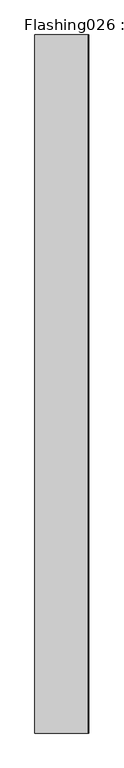
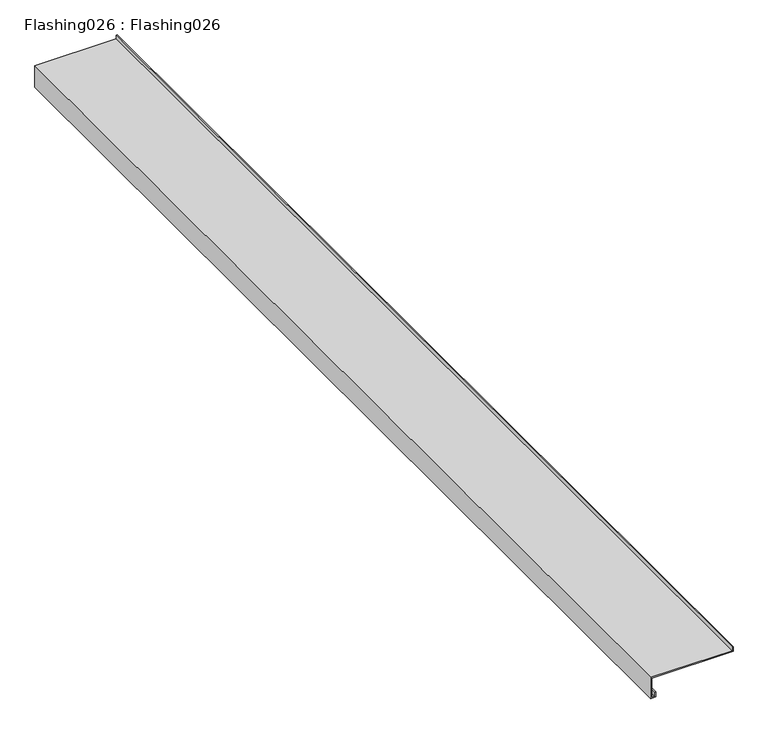
"""IFC4 building model written with IfcOpenShell, lengths in millimetres: proxy geometry, Flashing026 : Flashing026."""

from ifc_helpers import new_model, si_unit, frame, origin, place, context, project, spatial, polyline, outline, extrude, source, transform, mapped, element, save


def flashing026_flashing026_3ad6fd26(model_context):
    return source(origin(), model_context, "Body", "SweptSolid", [
        extrude(outline(polyline([(36566.1804687, -1997.9650879), (36558.9851563, -1997.9650879), (36558.9851563, -2150.7495117), (36516.8054688, -2150.7495117), (36516.8054688, -2140.6896973), (36527.3601562, -2140.6896973), (36527.3601562, -2142.6896973), (36518.8054687, -2142.6896973), (36518.8054687, -2148.7495117), (36556.9851562, -2148.7495117), (36556.9851562, -1995.9650879), (36566.1804687, -1995.9650879), (36566.1804687, -1997.9650879)])), frame((0.0, 998.1570053, 0.0), z_axis=(0.0, 1.0, 0.0), x_axis=(0.0, 0.0, 1.0)), (0.0, 0.0, 1.0), 2000.0),
    ])


if __name__ == "__main__":
    model = new_model("IFC4")
    model_context = context("Model", 3, world=origin())
    ifc_project = project(units=[si_unit("LENGTHUNIT", "METRE", prefix="MILLI")], contexts=[model_context])
    site = spatial("IfcSite", under=ifc_project)
    building = spatial("IfcBuilding", under=site)
    placement = place(None, origin())
    flashing026_flashing026_shape = flashing026_flashing026_3ad6fd26(model_context)
    element("IfcBuildingElementProxy", 1, Name="Flashing026 : Flashing026", ObjectType="Flashing026 : Flashing026", at=placement, inside=building, context=model_context, shape_type="MappedRepresentation", body=[
        mapped(flashing026_flashing026_shape, transform((0.0, 0.0, 0.0), x_axis=(1.0, 0.0, 0.0), y_axis=(0.0, 1.0, 0.0), z_axis=(0.0, 0.0, 1.0))),
    ])
    save(model, "model.ifc")

# Revit data of these elements
# Type "Flashing026 : Flashing026"
#   NameOverride = "Flashing026"
# Element 1 (IfcBuildingElementProxy, "Flashing026 : Flashing026")
#   Materials on its faces: "COPPER SILL PAN AT ALL EXTERIOR WINDOWS/DOORS PER DETAIL 1/A4.1"
# Materials
#   "COPPER SILL PAN AT ALL EXTERIOR WINDOWS/DOORS PER DETAIL 1/A4.1": class "Unassigned", colour RGB 255 170 255, transparency 0, Cost = 0
